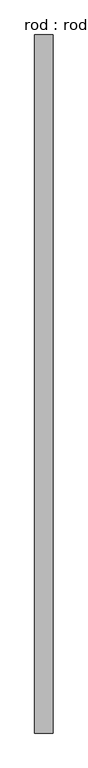
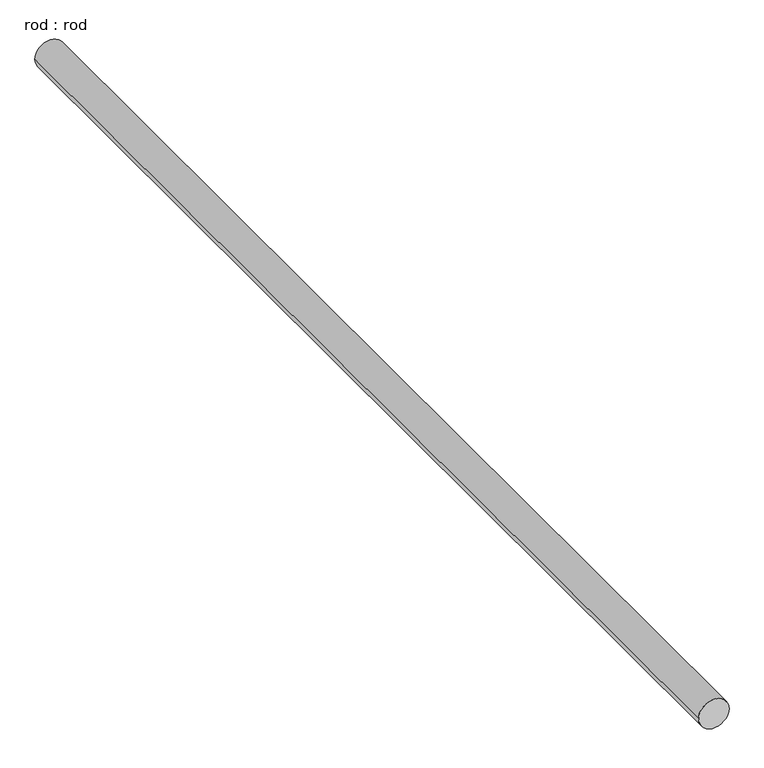
"""IFC4 building model written with IfcOpenShell, lengths in millimetres: proxy geometry, rod : rod."""

from ifc_helpers import new_model, si_unit, point, frame, frame_2d, origin, place, context, project, spatial, circle_curve, trimmed, segment, composite_curve, outline, extrude, source, transform, mapped, element, save


def rod_rod_29761a59(model_context):
    return source(origin(), model_context, "Body", "SweptSolid", [
        extrude(outline(composite_curve([segment(trimmed(circle_curve(frame_2d((0.0108462, 0.0)), 200.0), [point((0.0108462, 200.0))], [point((0.0108462, -200.0))], False, "CARTESIAN"), True, "CONTINUOUS"), segment(trimmed(circle_curve(frame_2d((0.0108462, 0.0)), 200.0), [point((0.0108462, -200.0))], [point((0.0108462, 200.0))], False, "CARTESIAN"), True, "CONTINUOUS")], self_intersect=False)), frame((0.0, -3471.3806156, 0.0), z_axis=(0.0, 1.0, 0.0), x_axis=(0.0, 0.0, 1.0)), (0.0, 0.0, 1.0), 15128.2184618),
    ])


if __name__ == "__main__":
    model = new_model("IFC4")
    model_context = context("Model", 3, world=origin())
    ifc_project = project(units=[si_unit("LENGTHUNIT", "METRE", prefix="MILLI")], contexts=[model_context])
    site = spatial("IfcSite", under=ifc_project)
    building = spatial("IfcBuilding", under=site)
    placement = place(None, origin())
    rod_rod_shape = rod_rod_29761a59(model_context)
    element("IfcBuildingElementProxy", 1, Name="rod : rod", ObjectType="rod : rod", at=placement, inside=building, context=model_context, shape_type="MappedRepresentation", body=[
        mapped(rod_rod_shape, transform((0.0, 0.0, 0.0), x_axis=(1.0, 0.0, 0.0), y_axis=(0.0, 1.0, 0.0), z_axis=(0.0, 0.0, 1.0))),
    ])
    save(model, "model.ifc")

# Revit data of these elements
# Type "rod : rod"
#   Default Elevation = 0
